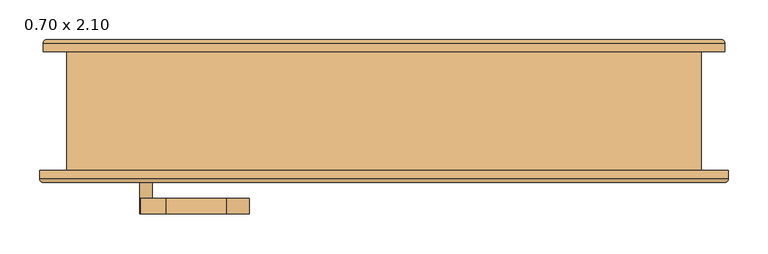
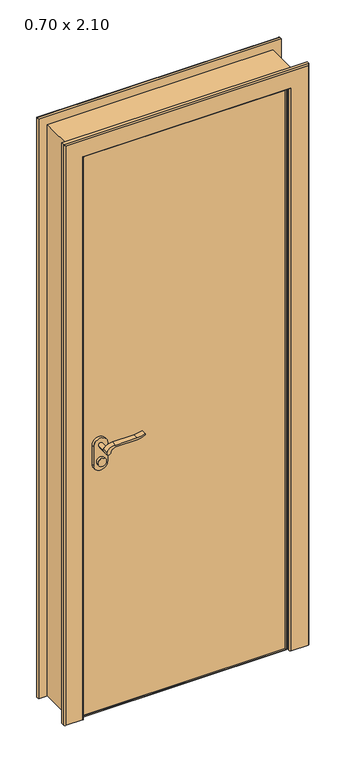
"""IFC4 building model written with IfcOpenShell, lengths in millimetres: door geometry, PORTA_DE_ABRIR_MADEIRA : 0.70 x 2.10."""

import ifcopenshell
import ifcopenshell.guid

model = None  # the IFC model being written
_history = None  # IfcOwnerHistory: only IFC2X3 demands one
_inside = {}  # id of a spatial element -> (the spatial element, [elements in it])
_under = {}  # id of a project, library or spatial element -> (it, [spatial elements below it])
_declared = {}  # id of a project -> (the project, [libraries it declares])
_typed = {}  # id of a type object -> (the type object, [elements of that type])
_made_of = {}  # id of a material, layer set ... -> (it, [elements and type objects made of it])


def new_model(schema):
    """Start an empty IFC model of exactly this schema.

    Asked for "IFC4X3", IfcOpenShell would pick the latest addendum, in which some entities
    have other attributes; the version numbers below select the first issue.
    IFC2X3 requires an IfcOwnerHistory on every rooted entity: one is made here for all.
    """
    global model, _history
    if schema == "IFC4X3":
        model = ifcopenshell.file(schema_version=(4, 3, 0, 0))
    else:
        model = ifcopenshell.file(schema=schema)
    _inside.clear()
    _under.clear()
    _declared.clear()
    _typed.clear()
    _made_of.clear()
    _history = None
    if model.schema == "IFC2X3":
        org = make("IfcOrganization", Name="unknown")
        user = make(
            "IfcPersonAndOrganization",
            ThePerson=make("IfcPerson", FamilyName="unknown"),
            TheOrganization=org,
        )
        app = make(
            "IfcApplication",
            ApplicationDeveloper=org,
            Version="unknown",
            ApplicationFullName="unknown",
            ApplicationIdentifier="unknown",
        )
        _history = make(
            "IfcOwnerHistory",
            OwningUser=user,
            OwningApplication=app,
            ChangeAction="ADDED",
            CreationDate=0,
        )
    return model


def make(cls, **values):
    """One entity of the class cls with the attributes given. An attribute that is None is left unset."""
    return model.create_entity(
        cls, **{name: value for name, value in values.items() if value is not None}
    )


def rooted(cls, **values):
    """An entity with a GlobalId (a new one), such as an element, a storey or a relation."""
    return make(cls, GlobalId=ifcopenshell.guid.new(), OwnerHistory=_history, **values)


def si_unit(unit_type, name, prefix=None):
    """IfcSIUnit, for example si_unit("LENGTHUNIT", "METRE", prefix="MILLI")."""
    return make("IfcSIUnit", UnitType=unit_type, Prefix=prefix, Name=name)


def assignment(units):
    """IfcUnitAssignment: the units of a project."""
    return None if units is None else make("IfcUnitAssignment", Units=units)


def point(xyz):
    """IfcCartesianPoint."""
    return None if xyz is None else make("IfcCartesianPoint", Coordinates=xyz)


def direction(xyz):
    """IfcDirection."""
    return None if xyz is None else make("IfcDirection", DirectionRatios=xyz)


def frame(location, z_axis=None, x_axis=None):
    """IfcAxis2Placement3D, a coordinate frame: its origin and axes. An axis left out is left unset."""
    return make(
        "IfcAxis2Placement3D",
        Location=point(location),
        Axis=direction(z_axis),
        RefDirection=direction(x_axis),
    )


def frame_2d(location, x_axis=None):
    """IfcAxis2Placement2D, a coordinate frame in the plane: its origin and x axis."""
    return make(
        "IfcAxis2Placement2D", Location=point(location), RefDirection=direction(x_axis)
    )


def origin():
    """The frame at (0, 0, 0) with its axes left unset."""
    return frame((0.0, 0.0, 0.0))


def origin_with_axes():
    """The frame at (0, 0, 0) with the z axis (0, 0, 1) and the x axis (1, 0, 0) written out."""
    return frame((0.0, 0.0, 0.0), z_axis=(0.0, 0.0, 1.0), x_axis=(1.0, 0.0, 0.0))


def place(relative_to, where):
    """IfcLocalPlacement: puts the frame where relative to a parent placement (None: the world)."""
    return make(
        "IfcLocalPlacement", PlacementRelTo=relative_to, RelativePlacement=where
    )


def context(
    kind, dimensions, precision=None, world=None, true_north=None, identifier=None
):
    """IfcGeometricRepresentationContext, for example the 3D "Model" context."""
    return make(
        "IfcGeometricRepresentationContext",
        ContextIdentifier=identifier,
        ContextType=kind,
        CoordinateSpaceDimension=dimensions,
        Precision=precision,
        WorldCoordinateSystem=world,
        TrueNorth=true_north,
    )


def project(units=None, contexts=None):
    """IfcProject with its units and contexts."""
    return rooted(
        "IfcProject",
        Name="project",
        RepresentationContexts=contexts,
        UnitsInContext=assignment(units),
    )


def spatial(cls, under=None, at=None, **own):
    """A site, building, storey or space (cls), placed at a placement, below another one or the project."""
    s = rooted(cls, ObjectPlacement=at, **own)
    if under is not None:
        _under.setdefault(under.id(), (under, []))[1].append(s)
    return s


def polyline(points):
    """IfcPolyline through the points."""
    return make("IfcPolyline", Points=[point(p) for p in points])


def circle_curve(where, radius):
    """IfcCircle in the frame where."""
    return make("IfcCircle", Position=where, Radius=radius)


def ellipse_curve(where, semi_axis1, semi_axis2):
    """IfcEllipse in the frame where."""
    return make(
        "IfcEllipse", Position=where, SemiAxis1=semi_axis1, SemiAxis2=semi_axis2
    )


def trimmed(basis, trim1, trim2, sense, master):
    """IfcTrimmedCurve: the piece of a basis curve between two trims."""
    return make(
        "IfcTrimmedCurve",
        BasisCurve=basis,
        Trim1=trim1,
        Trim2=trim2,
        SenseAgreement=sense,
        MasterRepresentation=master,
    )


def segment(curve, same_sense, transition):
    """IfcCompositeCurveSegment."""
    return make(
        "IfcCompositeCurveSegment",
        Transition=transition,
        SameSense=same_sense,
        ParentCurve=curve,
    )


def composite_curve(segments, self_intersect=None):
    """IfcCompositeCurve: segments joined end to end."""
    return make("IfcCompositeCurve", Segments=segments, SelfIntersect=self_intersect)


def outline(outer, holes=None, kind="AREA"):
    """IfcArbitraryClosedProfileDef: a profile drawn as a closed curve; with holes, ...WithVoids."""
    if holes is None:
        return make("IfcArbitraryClosedProfileDef", ProfileType=kind, OuterCurve=outer)
    return make(
        "IfcArbitraryProfileDefWithVoids",
        ProfileType=kind,
        OuterCurve=outer,
        InnerCurves=holes,
    )


def extrude(swept, where, along, depth):
    """IfcExtrudedAreaSolid: the profile swept, set in the frame where, extruded along a direction by depth."""
    return make(
        "IfcExtrudedAreaSolid",
        SweptArea=swept,
        Position=where,
        ExtrudedDirection=direction(along),
        Depth=depth,
    )


def faces_of(points, faces, orient=None, outer=None):
    """IfcFace entities. A face is a list of loops; a loop is a list of indices into points, from 0.

    orient and outer hold one flag for each loop. By default every Orientation is true, the
    first loop of a face is its IfcFaceOuterBound and the others are IfcFaceBound.
    """
    made = []
    for i, loops in enumerate(faces):
        bounds = []
        for j, loop in enumerate(loops):
            is_outer = j == 0 if outer is None else outer[i][j]
            bounds.append(
                make(
                    "IfcFaceOuterBound" if is_outer else "IfcFaceBound",
                    Bound=make("IfcPolyLoop", Polygon=[points[k] for k in loop]),
                    Orientation=True if orient is None else orient[i][j],
                )
            )
        made.append(make("IfcFace", Bounds=bounds))
    return made


def faceted_brep(points, faces, orient=None, outer=None, voids=None):
    """IfcFacetedBrep: a solid bounded by flat faces; with voids (closed shells), ...WithVoids."""
    shared = [point(p) for p in points]
    hull = make("IfcClosedShell", CfsFaces=faces_of(shared, faces, orient, outer))
    if voids is None:
        return make("IfcFacetedBrep", Outer=hull)
    return make(
        "IfcFacetedBrepWithVoids",
        Outer=hull,
        Voids=[
            make(cls, CfsFaces=faces_of(shared, fs, o, b)) for cls, fs, o, b in voids
        ],
    )


def shape(context_of_items, identifier, shape_type, items):
    """IfcShapeRepresentation: the items that make up one representation, for example the "Body"."""
    return make(
        "IfcShapeRepresentation",
        ContextOfItems=context_of_items,
        RepresentationIdentifier=identifier,
        RepresentationType=shape_type,
        Items=items,
    )


def source(mapping_origin, context_of_items, identifier, shape_type, items):
    """IfcRepresentationMap: a shape defined once, which mapped items show again and again."""
    return make(
        "IfcRepresentationMap",
        MappingOrigin=mapping_origin,
        MappedRepresentation=shape(context_of_items, identifier, shape_type, items),
    )


def transform(
    local_origin,
    x_axis=None,
    y_axis=None,
    z_axis=None,
    scale=None,
    scale2=None,
    scale3=None,
    uniform=True,
):
    """IfcCartesianTransformationOperator3D, or its non-uniform kind. x_axis, y_axis, z_axis: its Axis1, 2, 3."""
    if uniform:
        return make(
            "IfcCartesianTransformationOperator3D",
            Axis1=direction(x_axis),
            Axis2=direction(y_axis),
            LocalOrigin=point(local_origin),
            Scale=scale,
            Axis3=direction(z_axis),
        )
    return make(
        "IfcCartesianTransformationOperator3DnonUniform",
        Axis1=direction(x_axis),
        Axis2=direction(y_axis),
        LocalOrigin=point(local_origin),
        Scale=scale,
        Axis3=direction(z_axis),
        Scale2=scale2,
        Scale3=scale3,
    )


def mapped(mapping_source, mapping_target):
    """IfcMappedItem: shows the shape of a source again, moved by a transform."""
    return make(
        "IfcMappedItem", MappingSource=mapping_source, MappingTarget=mapping_target
    )


def made_of(thing, what):
    """Note that an element or type object is made of a material, layer set ...; save() writes the relation."""
    if what is not None:
        _made_of.setdefault(what.id(), (what, []))[1].append(thing)
    return thing


def element(
    cls,
    number,
    at=None,
    inside=None,
    cuts=None,
    type_object=None,
    material=None,
    context=None,
    identifier="Body",
    shape_type=None,
    held_by="IfcProductDefinitionShape",
    body=None,
    shapes=None,
    **own,
):
    """One element of the class cls, such as IfcWall. Its Tag is "e" and its number.

    at: its placement. inside: the storey or other place that contains it. cuts: it is an
    opening in that element (IfcRelVoidsElement). A single representation is given by context,
    identifier, shape_type and body (its items); several are given by shapes. held_by: the class
    of the entity that holds the representations. save() writes the other relations.
    """
    e = rooted(cls, Tag="e%d" % number, ObjectPlacement=at, **own)
    if body is not None:
        shapes = [shape(context, identifier, shape_type, body)]
    if shapes is not None:
        e.Representation = make(held_by, Representations=shapes)
    if inside is not None:
        _inside.setdefault(inside.id(), (inside, []))[1].append(e)
    if cuts is not None:
        rooted(
            "IfcRelVoidsElement", RelatingBuildingElement=cuts, RelatedOpeningElement=e
        )
    if type_object is not None:
        _typed.setdefault(type_object.id(), (type_object, []))[1].append(e)
    return made_of(e, material)


def aggregate(whole, parts):
    """IfcRelAggregates: a whole, such as a stair, and the parts it consists of."""
    return rooted("IfcRelAggregates", RelatingObject=whole, RelatedObjects=parts)


def save(model, path):
    """Write the relations noted so far, then the file.

    IfcRelAggregates (storeys below a building ...), IfcRelContainedInSpatialStructure (elements
    in a storey), IfcRelDefinesByType, IfcRelAssociatesMaterial and IfcRelDeclares: one each for
    every whole, place, type object, material and project.
    """
    for whole, parts in _under.values():
        aggregate(whole, parts)
    for where, things in _inside.values():
        rooted(
            "IfcRelContainedInSpatialStructure",
            RelatedElements=things,
            RelatingStructure=where,
        )
    for kind, things in _typed.values():
        rooted("IfcRelDefinesByType", RelatedObjects=things, RelatingType=kind)
    for what, things in _made_of.values():
        rooted("IfcRelAssociatesMaterial", RelatedObjects=things, RelatingMaterial=what)
    for by, libraries in _declared.values():
        rooted("IfcRelDeclares", RelatingContext=by, RelatedDefinitions=libraries)
    model.write(path)


def plane_surface(at):
    """IfcPlane: the flat surface through the origin of the frame at, square to its z axis."""
    return make("IfcPlane", Position=at)


def cylinder_surface(at, radius):
    """IfcCylindricalSurface: all points at the distance radius from the z axis of the frame at."""
    return make("IfcCylindricalSurface", Position=at, Radius=radius)


def advanced_brep(points, edges, surfaces, faces):
    """IfcAdvancedBrep: a solid bounded by faces that lie on surfaces and meet in shared edges.

    An edge is (start, end): straight between two places in points (the first is 0);
    or (start, end, curve); or (start, end, curve, False) where it runs against its curve.
    A face is (place in surfaces, loops), or (place, loops, False) where it looks against
    its surface's normal. A loop lists edges by number (the first is 1), with a minus sign
    where the edge is run from its end to its start. The first loop is the outer one.
    """
    corners = [point(p) for p in points]
    vertices = [make("IfcVertexPoint", VertexGeometry=c) for c in corners]
    made = []
    for start, end, *more in edges:
        made.append(
            make(
                "IfcEdgeCurve",
                EdgeStart=vertices[start],
                EdgeEnd=vertices[end],
                EdgeGeometry=more[0] if more else make("IfcPolyline", Points=[corners[start], corners[end]]),
                SameSense=more[1] if len(more) > 1 else True,
            )
        )
    hull = []
    for where, loops, *sense in faces:
        bounds = []
        for j, loop in enumerate(loops):
            ring = [make("IfcOrientedEdge", EdgeElement=made[abs(k) - 1], Orientation=k > 0) for k in loop]
            bounds.append(
                make(
                    "IfcFaceOuterBound" if j == 0 else "IfcFaceBound",
                    Bound=make("IfcEdgeLoop", EdgeList=ring),
                    Orientation=True,
                )
            )
        hull.append(make("IfcAdvancedFace", Bounds=bounds, FaceSurface=surfaces[where], SameSense=sense[0] if sense else True))
    return make("IfcAdvancedBrep", Outer=make("IfcClosedShell", CfsFaces=hull))


def door_0_70_x_2_10_a1a75d09(model_context):
    return source(origin(), model_context, "Body", "SolidModel", [
        extrude(outline(composite_curve([segment(trimmed(circle_curve(frame_2d((940.0, -300.0)), 15.0), [point((940.0, -285.0))], [point((940.0, -315.0))], False, "CARTESIAN"), True, "CONTINUOUS"), segment(trimmed(circle_curve(frame_2d((940.0, -300.0)), 15.0), [point((940.0, -315.0))], [point((940.0, -285.0))], False, "CARTESIAN"), True, "CONTINUOUS")], self_intersect=False)), frame((0.0, -25.0, 0.0), z_axis=(0.0, 1.0, 0.0), x_axis=(0.0, 0.0, 1.0)), (0.0, 0.0, 1.0), 10.0),
        extrude(outline(composite_curve([segment(trimmed(circle_curve(frame_2d((940.0, -300.0)), 15.0), [point((940.0, -285.0))], [point((940.0, -315.0))], False, "CARTESIAN"), True, "CONTINUOUS"), segment(trimmed(circle_curve(frame_2d((940.0, -300.0)), 15.0), [point((940.0, -315.0))], [point((940.0, -285.0))], False, "CARTESIAN"), True, "CONTINUOUS")], self_intersect=False)), frame((0.0, -90.0, 0.0), z_axis=(0.0, 1.0, 0.0), x_axis=(0.0, 0.0, 1.0)), (0.0, 0.0, 1.0), 10.0),
        extrude(outline(composite_curve([segment(trimmed(circle_curve(frame_2d((1000.0, -300.0)), 8.0), [point((1004.6523287, -306.5081363))], [point((1000.0, -292.0))], False, "CARTESIAN"), True, "CONTINUOUS"), segment(trimmed(circle_curve(frame_2d((994.8738613, -274.6138099)), 18.1261387), [point((1000.0, -292.0))], [point((1013.0, -274.6138099))], True, "CARTESIAN"), True, "CONTINUOUS"), segment(polyline([(1013.0, -274.6138099), (1013.0, -198.3564091)]), True, "CONTINUOUS"), segment(trimmed(circle_curve(frame_2d((1072.2709207, -201.9396612)), 59.3791355), [point((1013.0, -198.3564091))], [point((1022.2135558, -170.0))], False, "CARTESIAN"), True, "CONTINUOUS"), segment(polyline([(1022.2135558, -170.0), (1025.0, -170.0)]), True, "CONTINUOUS"), segment(trimmed(circle_curve(frame_2d((1103.2850638, -198.4227909)), 83.2850902), [point((1025.0, -170.0))], [point((1020.0, -198.3564091))], True, "CARTESIAN"), True, "CONTINUOUS"), segment(polyline([(1020.0, -198.3564091), (1020.0, -274.6325667)]), True, "CONTINUOUS"), segment(trimmed(circle_curve(frame_2d((982.7555521, -276.3324871)), 37.2832219), [point((1020.0, -274.6325667))], [point((1004.6523287, -306.5081363))], False, "CARTESIAN"), True, "CONTINUOUS")], self_intersect=False)), frame((0.0, 5.0, 0.0), z_axis=(0.0, 1.0, 0.0), x_axis=(0.0, 0.0, 1.0)), (0.0, 0.0, 1.0), 20.0),
        extrude(outline(composite_curve([segment(trimmed(circle_curve(frame_2d((994.8738682, -274.6138122)), 18.1261318), [point((999.9999903, -292.0))], [point((1013.0, -274.6138122))], True, "CARTESIAN"), True, "CONTINUOUS"), segment(polyline([(1013.0, -274.6138122), (1013.0, -198.3564091)]), True, "CONTINUOUS"), segment(trimmed(circle_curve(frame_2d((1072.2709207, -201.9396612)), 59.3791355), [point((1013.0, -198.3564091))], [point((1022.2135558, -170.0))], False, "CARTESIAN"), True, "CONTINUOUS"), segment(polyline([(1022.2135558, -170.0), (1025.0, -170.0)]), True, "CONTINUOUS"), segment(trimmed(circle_curve(frame_2d((1103.2850638, -198.4227909)), 83.2850902), [point((1025.0, -170.0))], [point((1020.0, -198.3564091))], True, "CARTESIAN"), True, "CONTINUOUS"), segment(polyline([(1020.0, -198.3564091), (1020.0, -274.6325667)]), True, "CONTINUOUS"), segment(trimmed(circle_curve(frame_2d((982.7555521, -276.3324871)), 37.2832219), [point((1020.0, -274.6325667))], [point((1004.6523287, -306.5081363))], False, "CARTESIAN"), True, "CONTINUOUS"), segment(trimmed(circle_curve(frame_2d((1000.0, -300.0)), 8.0), [point((1004.6523287, -306.5081363))], [point((999.9999903, -292.0))], False, "CARTESIAN"), True, "CONTINUOUS")], self_intersect=False)), frame((0.0, -130.0, 0.0), z_axis=(0.0, 1.0, 0.0), x_axis=(0.0, 0.0, 1.0)), (0.0, 0.0, 1.0), 20.0),
        extrude(outline(composite_curve([segment(trimmed(circle_curve(frame_2d((1000.0, -300.0)), 8.0), [point((1000.0, -292.0))], [point((1000.0, -308.0))], False, "CARTESIAN"), True, "CONTINUOUS"), segment(trimmed(circle_curve(frame_2d((1000.0, -300.0)), 8.0), [point((1000.0, -308.0))], [point((1000.0, -292.0))], False, "CARTESIAN"), True, "CONTINUOUS")], self_intersect=False)), frame((0.0, -25.0, 0.0), z_axis=(0.0, 1.0, 0.0), x_axis=(0.0, 0.0, 1.0)), (0.0, 0.0, 1.0), 30.0),
        extrude(outline(composite_curve([segment(trimmed(circle_curve(frame_2d((1000.0, -300.0)), 8.0), [point((1000.0, -292.0))], [point((1000.0, -308.0))], False, "CARTESIAN"), True, "CONTINUOUS"), segment(trimmed(circle_curve(frame_2d((1000.0, -300.0)), 8.0), [point((1000.0, -308.0))], [point((1000.0, -292.0))], False, "CARTESIAN"), True, "CONTINUOUS")], self_intersect=False)), frame((0.0, -110.0, 0.0), z_axis=(0.0, 1.0, 0.0), x_axis=(0.0, 0.0, 1.0)), (0.0, 0.0, 1.0), 30.0),
        extrude(outline(composite_curve([segment(trimmed(circle_curve(frame_2d((930.0, -300.0)), 25.0), [point((930.0, -325.0))], [point((930.0, -275.0))], False, "CARTESIAN"), True, "CONTINUOUS"), segment(polyline([(930.0, -275.0), (1000.0, -275.0)]), True, "CONTINUOUS"), segment(trimmed(circle_curve(frame_2d((1000.0, -300.0)), 25.0), [point((1000.0, -275.0))], [point((1000.0, -325.0))], False, "CARTESIAN"), True, "CONTINUOUS"), segment(polyline([(1000.0, -325.0), (930.0, -325.0)]), True, "CONTINUOUS")], self_intersect=False)), frame((0.0, -35.0, 0.0), z_axis=(0.0, 1.0, 0.0), x_axis=(0.0, 0.0, 1.0)), (0.0, 0.0, 1.0), 10.0),
        extrude(outline(composite_curve([segment(trimmed(circle_curve(frame_2d((930.0, -300.0)), 25.0), [point((930.0, -325.0))], [point((930.0, -275.0))], False, "CARTESIAN"), True, "CONTINUOUS"), segment(polyline([(930.0, -275.0), (1000.0, -275.0)]), True, "CONTINUOUS"), segment(trimmed(circle_curve(frame_2d((1000.0, -300.0)), 25.0), [point((1000.0, -275.0))], [point((1000.0, -325.0))], False, "CARTESIAN"), True, "CONTINUOUS"), segment(polyline([(1000.0, -325.0), (930.0, -325.0)]), True, "CONTINUOUS")], self_intersect=False)), frame((0.0, -80.0, 0.0), z_axis=(0.0, 1.0, 0.0), x_axis=(0.0, 0.0, 1.0)), (0.0, 0.0, 1.0), 10.0),
        faceted_brep([(-360.0, -35.0, 0.0), (-360.0, -75.0, 0.0), (-400.0, -75.0, 0.0), (-400.0, 75.0, 0.0), (-350.0, 75.0, 0.0), (-350.0, -35.0, 0.0), (-360.0, -35.0, 2100.0), (-360.0, -75.0, 2100.0), (360.0, -75.0, 2100.0), (360.0, -75.0, 0.0), (400.0, -75.0, 0.0), (400.0, -75.0, 2140.0), (-400.0, -75.0, 2140.0), (-400.0, 75.0, 2140.0), (400.0, 75.0, 2140.0), (400.0, 75.0, 0.0), (350.0, 75.0, 0.0), (350.0, 75.0, 2090.0), (-350.0, 75.0, 2090.0), (-350.0, -35.0, 2090.0), (350.0, -35.0, 2090.0), (350.0, -35.0, 0.0), (360.0, -35.0, 0.0), (360.0, -35.0, 2100.0)], [[[0, 1, 2, 3, 4, 5]], [[1, 0, 6, 7]], [[2, 1, 7, 8, 9, 10, 11, 12]], [[3, 2, 12, 13]], [[4, 3, 13, 14, 15, 16, 17, 18]], [[5, 4, 18, 19]], [[0, 5, 19, 20, 21, 22, 23, 6]], [[20, 17, 16, 21]], [[22, 21, 16, 15, 10, 9]], [[8, 23, 22, 9]], [[14, 11, 10, 15]], [[13, 12, 11, 14]], [[19, 18, 17, 20]], [[7, 6, 23, 8]]]),
        advanced_brep(
        [(-430.0, 75.3, 0.0), (-430.0, 85.3, 0.0), (-425.0, 90.3, 0.0), (-365.0, 90.3, 0.0), (-360.0, 85.3, 0.0), (-360.0, 75.3, 0.0), (-430.0, 75.3, 2170.0), (-430.0, 85.3, 2170.0), (-425.0, 90.3, 2165.0), (425.0, 90.3, 2165.0), (425.0, 90.3, 0.0), (365.0, 90.3, 0.0), (365.0, 90.3, 2105.0), (-365.0, 90.3, 2105.0), (-360.0, 85.3, 2100.0), (-360.0, 75.3, 2100.0), (360.0, 75.3, 2100.0), (360.0, 75.3, 0.0), (430.0, 75.3, 0.0), (430.0, 75.3, 2170.0), (360.0, 85.3, 0.0), (430.0, 85.3, 0.0), (360.0, 85.3, 2100.0), (430.0, 85.3, 2170.0)],
        [
            (0, 1),
            (1, 2, circle_curve(frame((-425.0, 85.3, 0.0), z_axis=(0.0, 0.0, -1.0), x_axis=(-1.0, 0.0, 0.0)), 5.0)),
            (2, 3),
            (3, 4, circle_curve(frame((-365.0, 85.3, 0.0), z_axis=(0.0, 0.0, -1.0), x_axis=(-1.0, 0.0, 0.0)), 5.0)),
            (4, 5),
            (5, 0),
            (0, 6),
            (6, 7),
            (7, 1),
            (7, 8, ellipse_curve(frame((-425.0, 85.3, 2165.0), z_axis=(-0.7071067811865475, 0.0, -0.7071067811865475), x_axis=(0.7071067811865474, 0.0, -0.7071067811865476)), 7.0710678, 5.0)),
            (8, 2),
            (8, 9),
            (9, 10),
            (10, 11),
            (11, 12),
            (12, 13),
            (13, 3),
            (13, 14, ellipse_curve(frame((-365.0, 85.3, 2105.0), z_axis=(-0.7071067811865475, 0.0, -0.7071067811865475), x_axis=(0.7071067811865474, 0.0, -0.7071067811865476)), 7.0710678, 5.0)),
            (14, 4),
            (14, 15),
            (15, 5),
            (15, 16),
            (16, 17),
            (17, 18),
            (18, 19),
            (19, 6),
            (17, 20),
            (20, 11, circle_curve(frame((365.0, 85.3, 0.0), z_axis=(0.0, 0.0, -1.0), x_axis=(1.0, 0.0, 0.0)), 5.0)),
            (10, 21, circle_curve(frame((425.0, 85.3, 0.0), z_axis=(0.0, 0.0, -1.0), x_axis=(1.0, 0.0, 0.0)), 5.0)),
            (21, 18),
            (16, 22),
            (22, 20),
            (22, 12, ellipse_curve(frame((365.0, 85.3, 2105.0), z_axis=(0.7071067811865475, 0.0, -0.7071067811865475), x_axis=(0.7071067811865474, 0.0, 0.7071067811865476)), 7.0710678, 5.0)),
            (9, 23, ellipse_curve(frame((425.0, 85.3, 2165.0), z_axis=(0.7071067811865475, 0.0, -0.7071067811865475), x_axis=(0.7071067811865474, 0.0, 0.7071067811865476)), 7.0710678, 5.0)),
            (23, 21),
            (23, 19),
            (23, 7),
            (14, 22),
        ],
        [
            plane_surface(frame((-400.0, -75.0, 0.0), z_axis=(0.0, 0.0, -1.0), x_axis=(0.0, -1.0, 0.0))),
            plane_surface(frame((-430.0, 75.3, 0.0), z_axis=(-1.0, 0.0, 0.0), x_axis=(0.0, 0.0, 1.0))),
            cylinder_surface(frame((-425.0, 85.3, 0.0), z_axis=(0.0, 0.0, -1.0), x_axis=(-1.0, 0.0, 0.0)), 5.0),
            plane_surface(frame((-425.0, 90.3, 0.0), z_axis=(0.0, 1.0, 0.0), x_axis=(0.0, 0.0, 1.0))),
            cylinder_surface(frame((-365.0, 85.3, 0.0), z_axis=(0.0, 0.0, -1.0), x_axis=(-1.0, 0.0, 0.0)), 5.0),
            plane_surface(frame((-360.0, 85.3, 0.0), z_axis=(1.0, 0.0, 0.0), x_axis=(0.0, 0.0, 1.0))),
            plane_surface(frame((-360.0, 75.3, 0.0), z_axis=(0.0, -1.0, 0.0), x_axis=(0.0, 0.0, 1.0))),
            plane_surface(frame((400.0, -75.0, 0.0), z_axis=(0.0, 0.0, -1.0), x_axis=(0.0, -1.0, 0.0))),
            plane_surface(frame((360.0, 85.3, 2100.0), z_axis=(-1.0, 0.0, 0.0), x_axis=(0.0, 0.0, -1.0))),
            cylinder_surface(frame((365.0, 85.3, 2140.0), z_axis=(0.0, 0.0, 1.0), x_axis=(1.0, 0.0, 0.0)), 5.0),
            cylinder_surface(frame((425.0, 85.3, 2140.0), z_axis=(0.0, 0.0, 1.0), x_axis=(1.0, 0.0, 0.0)), 5.0),
            plane_surface(frame((430.0, 75.3, 2170.0), z_axis=(1.0, 0.0, 0.0), x_axis=(0.0, 0.0, -1.0))),
            plane_surface(frame((-430.0, 75.3, 2170.0), z_axis=(0.0, 0.0, 1.0), x_axis=(1.0, 0.0, 0.0))),
            plane_surface(frame((-360.0, 85.3, 2100.0), z_axis=(0.0, 0.0, -1.0), x_axis=(1.0, 0.0, 0.0))),
            cylinder_surface(frame((-400.0, 85.3, 2165.0), z_axis=(-1.0, 0.0, 0.0), x_axis=(0.0, 0.0, 1.0)), 5.0),
            cylinder_surface(frame((-400.0, 85.3, 2105.0), z_axis=(-1.0, 0.0, 0.0), x_axis=(0.0, 0.0, 1.0)), 5.0),
        ],
        [
            (0, [[1, 2, 3, 4, 5, 6]]),
            (1, [[-1, 7, 8, 9]]),
            (2, [[-2, -9, 10, 11]]),
            (3, [[-3, -11, 12, 13, 14, 15, 16, 17]]),
            (4, [[-4, -17, 18, 19]]),
            (5, [[-5, -19, 20, 21]]),
            (6, [[-6, -21, 22, 23, 24, 25, 26, -7]]),
            (7, [[-24, 27, 28, -14, 29, 30]]),
            (8, [[31, 32, -27, -23]]),
            (9, [[33, -15, -28, -32]]),
            (10, [[34, 35, -29, -13]]),
            (11, [[36, -25, -30, -35]]),
            (12, [[-8, -26, -36, 37]]),
            (13, [[-20, 38, -31, -22]]),
            (14, [[-10, -37, -34, -12]]),
            (15, [[-18, -16, -33, -38]]),
        ],
    ),
        advanced_brep(
        [(-429.3155593, -90.2647517, 0.0), (-434.3155593, -85.2647517, 0.0), (-434.3155593, -75.2647517, 0.0), (-364.3155593, -75.2647517, 0.0), (-364.3155593, -85.2647517, 0.0), (-369.3155593, -90.2647517, 0.0), (-429.3155593, -90.2647517, 2169.3155593), (-434.3155593, -85.2647517, 2174.3155593), (-434.3155593, -75.2647517, 2174.3155593), (434.3155593, -75.2647517, 2174.3155593), (434.3155593, -75.2647517, 0.0), (364.3155593, -75.2647517, 0.0), (364.3155593, -75.2647517, 2104.3155593), (-364.3155593, -75.2647517, 2104.3155593), (-364.3155593, -85.2647517, 2104.3155593), (-369.3155593, -90.2647517, 2109.3155593), (369.3155593, -90.2647517, 2109.3155593), (369.3155593, -90.2647517, 0.0), (429.3155593, -90.2647517, 0.0), (429.3155593, -90.2647517, 2169.3155593), (364.3155593, -85.2647517, 0.0), (434.3155593, -85.2647517, 0.0), (364.3155593, -85.2647517, 2104.3155593), (434.3155593, -85.2647517, 2174.3155593)],
        [
            (0, 1, circle_curve(frame((-429.3155593, -85.2647517, 0.0), z_axis=(0.0, 0.0, -1.0), x_axis=(-1.0, 0.0, 0.0)), 5.0)),
            (1, 2),
            (2, 3),
            (3, 4),
            (4, 5, circle_curve(frame((-369.3155593, -85.2647517, 0.0), z_axis=(0.0, 0.0, -1.0), x_axis=(-1.0, 0.0, 0.0)), 5.0)),
            (5, 0),
            (0, 6),
            (6, 7, ellipse_curve(frame((-429.3155593, -85.2647517, 2169.3155593), z_axis=(-0.7071067811865475, 0.0, -0.7071067811865475), x_axis=(0.7071067811865474, 0.0, -0.7071067811865476)), 7.0710678, 5.0)),
            (7, 1),
            (7, 8),
            (8, 2),
            (8, 9),
            (9, 10),
            (10, 11),
            (11, 12),
            (12, 13),
            (13, 3),
            (13, 14),
            (14, 4),
            (14, 15, ellipse_curve(frame((-369.3155593, -85.2647517, 2109.3155593), z_axis=(-0.7071067811865475, 0.0, -0.7071067811865475), x_axis=(0.7071067811865474, 0.0, -0.7071067811865476)), 7.0710678, 5.0)),
            (15, 5),
            (15, 16),
            (16, 17),
            (17, 18),
            (18, 19),
            (19, 6),
            (17, 20, circle_curve(frame((369.3155593, -85.2647517, 0.0), z_axis=(0.0, 0.0, -1.0), x_axis=(1.0, 0.0, 0.0)), 5.0)),
            (20, 11),
            (10, 21),
            (21, 18, circle_curve(frame((429.3155593, -85.2647517, 0.0), z_axis=(0.0, 0.0, -1.0), x_axis=(1.0, 0.0, 0.0)), 5.0)),
            (16, 22, ellipse_curve(frame((369.3155593, -85.2647517, 2109.3155593), z_axis=(0.7071067811865475, 0.0, -0.7071067811865475), x_axis=(0.7071067811865474, 0.0, 0.7071067811865476)), 7.0710678, 5.0)),
            (22, 20),
            (22, 12),
            (9, 23),
            (23, 21),
            (23, 19, ellipse_curve(frame((429.3155593, -85.2647517, 2169.3155593), z_axis=(0.7071067811865475, 0.0, -0.7071067811865475), x_axis=(0.7071067811865474, 0.0, 0.7071067811865476)), 7.0710678, 5.0)),
            (7, 23),
            (22, 14),
        ],
        [
            plane_surface(frame((-400.0, -75.0, 0.0), z_axis=(0.0, 0.0, -1.0), x_axis=(0.0, -1.0, 0.0))),
            cylinder_surface(frame((-429.3155593, -85.2647517, 0.0), z_axis=(0.0, 0.0, -1.0), x_axis=(-1.0, 0.0, 0.0)), 5.0),
            plane_surface(frame((-434.3155593, -85.2647517, 0.0), z_axis=(-1.0, 0.0, 0.0), x_axis=(0.0, 0.0, 1.0))),
            plane_surface(frame((-434.3155593, -75.2647517, 0.0), z_axis=(0.0, 1.0, 0.0), x_axis=(0.0, 0.0, 1.0))),
            plane_surface(frame((-364.3155593, -75.2647517, 0.0), z_axis=(1.0, 0.0, 0.0), x_axis=(0.0, 0.0, 1.0))),
            cylinder_surface(frame((-369.3155593, -85.2647517, 0.0), z_axis=(0.0, 0.0, -1.0), x_axis=(-1.0, 0.0, 0.0)), 5.0),
            plane_surface(frame((-369.3155593, -90.2647517, 0.0), z_axis=(0.0, -1.0, 0.0), x_axis=(0.0, 0.0, 1.0))),
            plane_surface(frame((400.0, -75.0, 0.0), z_axis=(0.0, 0.0, -1.0), x_axis=(0.0, -1.0, 0.0))),
            cylinder_surface(frame((369.3155593, -85.2647517, 2140.0), z_axis=(0.0, 0.0, 1.0), x_axis=(1.0, 0.0, 0.0)), 5.0),
            plane_surface(frame((364.3155593, -75.2647517, 2104.3155593), z_axis=(-1.0, 0.0, 0.0), x_axis=(0.0, 0.0, -1.0))),
            plane_surface(frame((434.3155593, -85.2647517, 2174.3155593), z_axis=(1.0, 0.0, 0.0), x_axis=(0.0, 0.0, -1.0))),
            cylinder_surface(frame((429.3155593, -85.2647517, 2140.0), z_axis=(0.0, 0.0, 1.0), x_axis=(1.0, 0.0, 0.0)), 5.0),
            plane_surface(frame((-434.3155593, -85.2647517, 2174.3155593), z_axis=(0.0, 0.0, 1.0), x_axis=(1.0, 0.0, 0.0))),
            plane_surface(frame((-364.3155593, -75.2647517, 2104.3155593), z_axis=(0.0, 0.0, -1.0), x_axis=(1.0, 0.0, 0.0))),
            cylinder_surface(frame((-400.0, -85.2647517, 2169.3155593), z_axis=(-1.0, 0.0, 0.0), x_axis=(0.0, 0.0, 1.0)), 5.0),
            cylinder_surface(frame((-400.0, -85.2647517, 2109.3155593), z_axis=(-1.0, 0.0, 0.0), x_axis=(0.0, 0.0, 1.0)), 5.0),
        ],
        [
            (0, [[1, 2, 3, 4, 5, 6]]),
            (1, [[-1, 7, 8, 9]]),
            (2, [[-2, -9, 10, 11]]),
            (3, [[-3, -11, 12, 13, 14, 15, 16, 17]]),
            (4, [[-4, -17, 18, 19]]),
            (5, [[-5, -19, 20, 21]]),
            (6, [[-6, -21, 22, 23, 24, 25, 26, -7]]),
            (7, [[-24, 27, 28, -14, 29, 30]]),
            (8, [[31, 32, -27, -23]]),
            (9, [[33, -15, -28, -32]]),
            (10, [[34, 35, -29, -13]]),
            (11, [[36, -25, -30, -35]]),
            (12, [[-10, 37, -34, -12]]),
            (13, [[-18, -16, -33, 38]]),
            (14, [[-8, -26, -36, -37]]),
            (15, [[-20, -38, -31, -22]]),
        ],
    ),
        extrude(outline(polyline([(360.0, -70.0), (-360.0, -70.0), (-360.0, -35.0), (360.0, -35.0), (360.0, -70.0)])), origin_with_axes(), (0.0, 0.0, 1.0), 2100.0),
        extrude(outline(polyline([(-350.0, -35.0), (-350.0, 75.0), (350.0, 75.0), (350.0, -35.0), (360.0, -35.0), (360.0, -75.0), (-360.0, -75.0), (-360.0, -35.0), (-350.0, -35.0)])), frame((0.0, 0.0, -3.0), z_axis=(0.0, 0.0, 1.0), x_axis=(1.0, 0.0, 0.0)), (0.0, 0.0, 1.0), 3.1),
    ])


if __name__ == "__main__":
    model = new_model("IFC4")
    model_context = context("Model", 3, world=origin())
    ifc_project = project(units=[si_unit("LENGTHUNIT", "METRE", prefix="MILLI")], contexts=[model_context])
    site = spatial("IfcSite", under=ifc_project)
    building = spatial("IfcBuilding", under=site)
    placement = place(None, origin())
    door_0_70_x_2_10_shape = door_0_70_x_2_10_a1a75d09(model_context)
    element("IfcDoor", 1, ObjectType="PORTA_DE_ABRIR_MADEIRA : 0.70 x 2.10", at=placement, inside=building, context=model_context, shape_type="MappedRepresentation", body=[
        mapped(door_0_70_x_2_10_shape, transform((0.0, 0.0, 0.0), x_axis=(1.0, 0.0, 0.0), y_axis=(0.0, 1.0, 0.0), z_axis=(0.0, 0.0, 1.0))),
    ])
    save(model, "model.ifc")

# Revit data of these elements
# Type "PORTA_DE_ABRIR_MADEIRA : 0.70 x 2.10"
#   Type Mark = "P3"
#   Analytic Construction = "<Nenhum>"
#   Rough Width = 0.80 m
#   Projeção da estrutura externa = 0.025 m
#   Projeção da estrutura interna = 0.025 m
#   Largura da estrutura = 0.075 m
#   Rough Height = 2.15 m
#   Height = 2.10 m
#   Width = 0.70 m
#   Soleira [instance default] = no
#   Material do batente = .BATENTE E GUARNIÇÃO
#   Material da maçaneta = .AÇO INOXIDÁVEL ESCOVADO
#   Material da folha da porta = .FOLHA DA PORTA
#   Material da Soleira [instance default] = none
#   Function = (empty or 0)
#   Wall Closure = (empty or 0)
# Element 1 (IfcDoor, "PORTA_DE_ABRIR_MADEIRA : 0.70 x 2.10")
#   Soleira = yes
#   Material da Soleira = .GRANITO BRANCO ITAUNAS
#   Materials on its faces: ".AÇO INOXIDÁVEL ESCOVADO", ".BATENTE E GUARNIÇÃO", ".GRANITO BRANCO ITAUNAS", ".FOLHA DA PORTA"
# Materials
#   ".BATENTE E GUARNIÇÃO": class "Madeira", colour RGB 215 186 156, transparency 0, Cost = 0
#   ".AÇO INOXIDÁVEL ESCOVADO": class "Metal", colour RGB 189 187 185, transparency 0, Description = "Stainless Steel 18/8, brushed finish", Cost = 0
#   ".FOLHA DA PORTA": class "Madeira", colour RGB 148 119 91, transparency 0, Cost = 0
#   ".GRANITO BRANCO ITAUNAS": class ".CC_PEDRA REVEST.", colour RGB 202 195 174, transparency 0, Description = "Revestimento em granito", Cost = 0
